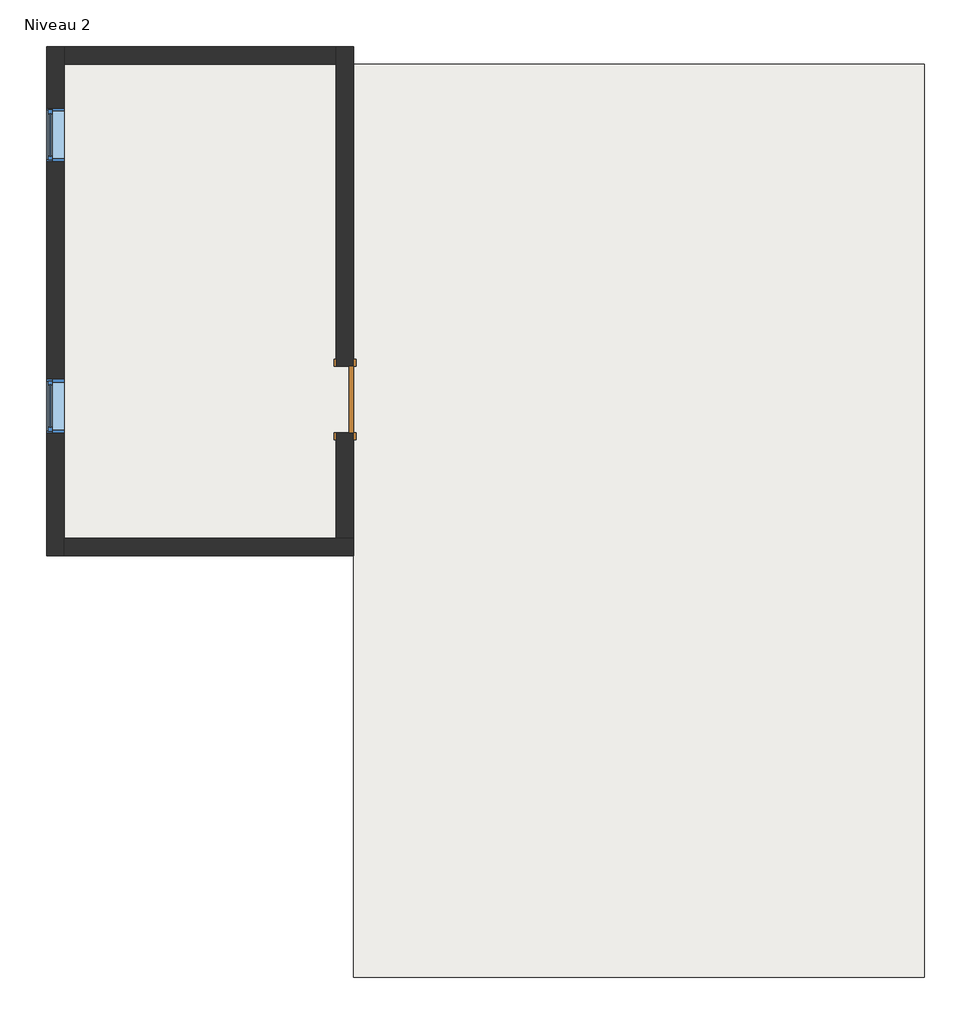
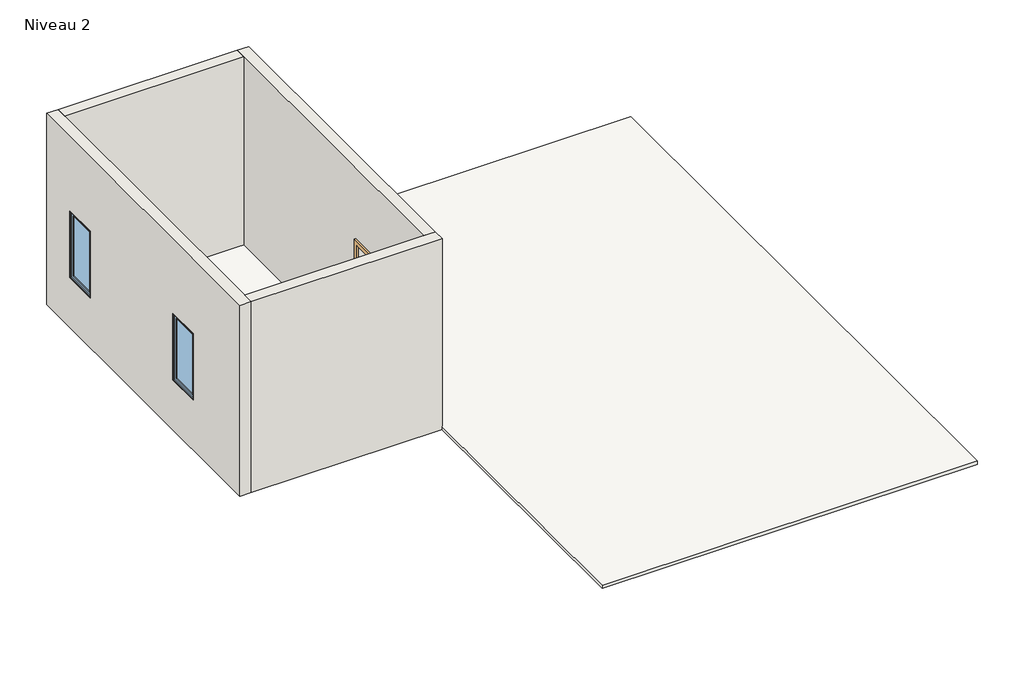
# One storey: 4 walls, 2 windows, 1 covering, 1 door.
"""IFC4 building model written with IfcOpenShell, lengths in millimetres."""

import ifcopenshell
import ifcopenshell.guid

model = None  # the IFC model being written
_history = None  # IfcOwnerHistory: only IFC2X3 demands one
_inside = {}  # id of a spatial element -> (the spatial element, [elements in it])
_under = {}  # id of a project, library or spatial element -> (it, [spatial elements below it])
_declared = {}  # id of a project -> (the project, [libraries it declares])
_typed = {}  # id of a type object -> (the type object, [elements of that type])
_made_of = {}  # id of a material, layer set ... -> (it, [elements and type objects made of it])


def new_model(schema):
    """Start an empty IFC model of exactly this schema.

    Asked for "IFC4X3", IfcOpenShell would pick the latest addendum, in which some entities
    have other attributes; the version numbers below select the first issue.
    IFC2X3 requires an IfcOwnerHistory on every rooted entity: one is made here for all.
    """
    global model, _history
    if schema == "IFC4X3":
        model = ifcopenshell.file(schema_version=(4, 3, 0, 0))
    else:
        model = ifcopenshell.file(schema=schema)
    _inside.clear()
    _under.clear()
    _declared.clear()
    _typed.clear()
    _made_of.clear()
    _history = None
    if model.schema == "IFC2X3":
        org = make("IfcOrganization", Name="unknown")
        user = make(
            "IfcPersonAndOrganization",
            ThePerson=make("IfcPerson", FamilyName="unknown"),
            TheOrganization=org,
        )
        app = make(
            "IfcApplication",
            ApplicationDeveloper=org,
            Version="unknown",
            ApplicationFullName="unknown",
            ApplicationIdentifier="unknown",
        )
        _history = make(
            "IfcOwnerHistory",
            OwningUser=user,
            OwningApplication=app,
            ChangeAction="ADDED",
            CreationDate=0,
        )
    return model


def make(cls, **values):
    """One entity of the class cls with the attributes given. An attribute that is None is left unset."""
    return model.create_entity(
        cls, **{name: value for name, value in values.items() if value is not None}
    )


def rooted(cls, **values):
    """An entity with a GlobalId (a new one), such as an element, a storey or a relation."""
    return make(cls, GlobalId=ifcopenshell.guid.new(), OwnerHistory=_history, **values)


def si_unit(unit_type, name, prefix=None):
    """IfcSIUnit, for example si_unit("LENGTHUNIT", "METRE", prefix="MILLI")."""
    return make("IfcSIUnit", UnitType=unit_type, Prefix=prefix, Name=name)


def assignment(units):
    """IfcUnitAssignment: the units of a project."""
    return None if units is None else make("IfcUnitAssignment", Units=units)


def point(xyz):
    """IfcCartesianPoint."""
    return None if xyz is None else make("IfcCartesianPoint", Coordinates=xyz)


def direction(xyz):
    """IfcDirection."""
    return None if xyz is None else make("IfcDirection", DirectionRatios=xyz)


def frame(location, z_axis=None, x_axis=None):
    """IfcAxis2Placement3D, a coordinate frame: its origin and axes. An axis left out is left unset."""
    return make(
        "IfcAxis2Placement3D",
        Location=point(location),
        Axis=direction(z_axis),
        RefDirection=direction(x_axis),
    )


def origin():
    """The frame at (0, 0, 0) with its axes left unset."""
    return frame((0.0, 0.0, 0.0))


def origin_with_axes():
    """The frame at (0, 0, 0) with the z axis (0, 0, 1) and the x axis (1, 0, 0) written out."""
    return frame((0.0, 0.0, 0.0), z_axis=(0.0, 0.0, 1.0), x_axis=(1.0, 0.0, 0.0))


def place(relative_to, where):
    """IfcLocalPlacement: puts the frame where relative to a parent placement (None: the world)."""
    return make(
        "IfcLocalPlacement", PlacementRelTo=relative_to, RelativePlacement=where
    )


def context(
    kind, dimensions, precision=None, world=None, true_north=None, identifier=None
):
    """IfcGeometricRepresentationContext, for example the 3D "Model" context."""
    return make(
        "IfcGeometricRepresentationContext",
        ContextIdentifier=identifier,
        ContextType=kind,
        CoordinateSpaceDimension=dimensions,
        Precision=precision,
        WorldCoordinateSystem=world,
        TrueNorth=true_north,
    )


def project(units=None, contexts=None):
    """IfcProject with its units and contexts."""
    return rooted(
        "IfcProject",
        Name="project",
        RepresentationContexts=contexts,
        UnitsInContext=assignment(units),
    )


def spatial(cls, under=None, at=None, **own):
    """A site, building, storey or space (cls), placed at a placement, below another one or the project."""
    s = rooted(cls, ObjectPlacement=at, **own)
    if under is not None:
        _under.setdefault(under.id(), (under, []))[1].append(s)
    return s


def polyline(points):
    """IfcPolyline through the points."""
    return make("IfcPolyline", Points=[point(p) for p in points])


def outline(outer, holes=None, kind="AREA"):
    """IfcArbitraryClosedProfileDef: a profile drawn as a closed curve; with holes, ...WithVoids."""
    if holes is None:
        return make("IfcArbitraryClosedProfileDef", ProfileType=kind, OuterCurve=outer)
    return make(
        "IfcArbitraryProfileDefWithVoids",
        ProfileType=kind,
        OuterCurve=outer,
        InnerCurves=holes,
    )


def extrude(swept, where, along, depth):
    """IfcExtrudedAreaSolid: the profile swept, set in the frame where, extruded along a direction by depth."""
    return make(
        "IfcExtrudedAreaSolid",
        SweptArea=swept,
        Position=where,
        ExtrudedDirection=direction(along),
        Depth=depth,
    )


def faces_of(points, faces, orient=None, outer=None):
    """IfcFace entities. A face is a list of loops; a loop is a list of indices into points, from 0.

    orient and outer hold one flag for each loop. By default every Orientation is true, the
    first loop of a face is its IfcFaceOuterBound and the others are IfcFaceBound.
    """
    made = []
    for i, loops in enumerate(faces):
        bounds = []
        for j, loop in enumerate(loops):
            is_outer = j == 0 if outer is None else outer[i][j]
            bounds.append(
                make(
                    "IfcFaceOuterBound" if is_outer else "IfcFaceBound",
                    Bound=make("IfcPolyLoop", Polygon=[points[k] for k in loop]),
                    Orientation=True if orient is None else orient[i][j],
                )
            )
        made.append(make("IfcFace", Bounds=bounds))
    return made


def faceted_brep(points, faces, orient=None, outer=None, voids=None):
    """IfcFacetedBrep: a solid bounded by flat faces; with voids (closed shells), ...WithVoids."""
    shared = [point(p) for p in points]
    hull = make("IfcClosedShell", CfsFaces=faces_of(shared, faces, orient, outer))
    if voids is None:
        return make("IfcFacetedBrep", Outer=hull)
    return make(
        "IfcFacetedBrepWithVoids",
        Outer=hull,
        Voids=[
            make(cls, CfsFaces=faces_of(shared, fs, o, b)) for cls, fs, o, b in voids
        ],
    )


def shape(context_of_items, identifier, shape_type, items):
    """IfcShapeRepresentation: the items that make up one representation, for example the "Body"."""
    return make(
        "IfcShapeRepresentation",
        ContextOfItems=context_of_items,
        RepresentationIdentifier=identifier,
        RepresentationType=shape_type,
        Items=items,
    )


def source(mapping_origin, context_of_items, identifier, shape_type, items):
    """IfcRepresentationMap: a shape defined once, which mapped items show again and again."""
    return make(
        "IfcRepresentationMap",
        MappingOrigin=mapping_origin,
        MappedRepresentation=shape(context_of_items, identifier, shape_type, items),
    )


def transform(
    local_origin,
    x_axis=None,
    y_axis=None,
    z_axis=None,
    scale=None,
    scale2=None,
    scale3=None,
    uniform=True,
):
    """IfcCartesianTransformationOperator3D, or its non-uniform kind. x_axis, y_axis, z_axis: its Axis1, 2, 3."""
    if uniform:
        return make(
            "IfcCartesianTransformationOperator3D",
            Axis1=direction(x_axis),
            Axis2=direction(y_axis),
            LocalOrigin=point(local_origin),
            Scale=scale,
            Axis3=direction(z_axis),
        )
    return make(
        "IfcCartesianTransformationOperator3DnonUniform",
        Axis1=direction(x_axis),
        Axis2=direction(y_axis),
        LocalOrigin=point(local_origin),
        Scale=scale,
        Axis3=direction(z_axis),
        Scale2=scale2,
        Scale3=scale3,
    )


def mapped(mapping_source, mapping_target):
    """IfcMappedItem: shows the shape of a source again, moved by a transform."""
    return make(
        "IfcMappedItem", MappingSource=mapping_source, MappingTarget=mapping_target
    )


def made_of(thing, what):
    """Note that an element or type object is made of a material, layer set ...; save() writes the relation."""
    if what is not None:
        _made_of.setdefault(what.id(), (what, []))[1].append(thing)
    return thing


def element(
    cls,
    number,
    at=None,
    inside=None,
    cuts=None,
    type_object=None,
    material=None,
    context=None,
    identifier="Body",
    shape_type=None,
    held_by="IfcProductDefinitionShape",
    body=None,
    shapes=None,
    **own,
):
    """One element of the class cls, such as IfcWall. Its Tag is "e" and its number.

    at: its placement. inside: the storey or other place that contains it. cuts: it is an
    opening in that element (IfcRelVoidsElement). A single representation is given by context,
    identifier, shape_type and body (its items); several are given by shapes. held_by: the class
    of the entity that holds the representations. save() writes the other relations.
    """
    e = rooted(cls, Tag="e%d" % number, ObjectPlacement=at, **own)
    if body is not None:
        shapes = [shape(context, identifier, shape_type, body)]
    if shapes is not None:
        e.Representation = make(held_by, Representations=shapes)
    if inside is not None:
        _inside.setdefault(inside.id(), (inside, []))[1].append(e)
    if cuts is not None:
        rooted(
            "IfcRelVoidsElement", RelatingBuildingElement=cuts, RelatedOpeningElement=e
        )
    if type_object is not None:
        _typed.setdefault(type_object.id(), (type_object, []))[1].append(e)
    return made_of(e, material)


def aggregate(whole, parts):
    """IfcRelAggregates: a whole, such as a stair, and the parts it consists of."""
    return rooted("IfcRelAggregates", RelatingObject=whole, RelatedObjects=parts)


def save(model, path):
    """Write the relations noted so far, then the file.

    IfcRelAggregates (storeys below a building ...), IfcRelContainedInSpatialStructure (elements
    in a storey), IfcRelDefinesByType, IfcRelAssociatesMaterial and IfcRelDeclares: one each for
    every whole, place, type object, material and project.
    """
    for whole, parts in _under.values():
        aggregate(whole, parts)
    for where, things in _inside.values():
        rooted(
            "IfcRelContainedInSpatialStructure",
            RelatedElements=things,
            RelatingStructure=where,
        )
    for kind, things in _typed.values():
        rooted("IfcRelDefinesByType", RelatedObjects=things, RelatingType=kind)
    for what, things in _made_of.values():
        rooted("IfcRelAssociatesMaterial", RelatedObjects=things, RelatingMaterial=what)
    for by, libraries in _declared.values():
        rooted("IfcRelDeclares", RelatingContext=by, RelatedDefinitions=libraries)
    model.write(path)


def simple_avec_alignement_0762_x_2134mm_85379237(model_context):
    return source(origin(), model_context, "Body", "SweptSolid", [
        extrude(outline(polyline([(2210.0, -457.0), (0.0, -457.0), (0.0, -381.0), (2134.0, -381.0), (2134.0, 381.0), (0.0, 381.0), (0.0, 457.0), (2210.0, 457.0), (2210.0, -457.0)])), frame((0.0, 100.0, 0.0), z_axis=(0.0, 1.0, 0.0), x_axis=(0.0, 0.0, 1.0)), (0.0, 0.0, 1.0), 25.0),
        extrude(outline(polyline([(2210.0, 457.0), (2210.0, -457.0), (0.0, -457.0), (0.0, -381.0), (2134.0, -381.0), (2134.0, 381.0), (0.0, 381.0), (0.0, 457.0), (2210.0, 457.0)])), frame((0.0, -125.0, 0.0), z_axis=(0.0, 1.0, 0.0), x_axis=(0.0, 0.0, 1.0)), (0.0, 0.0, 1.0), 25.0),
        extrude(outline(polyline([(381.0, 49.0), (-381.0, 49.0), (-381.0, 100.0), (381.0, 100.0), (381.0, 49.0)])), origin_with_axes(), (0.0, 0.0, 1.0), 2134.0),
    ])


def fixe_0610_x_1220mm_4e981104(model_context):
    return source(origin(), model_context, "Body", "SweptSolid", [
        extrude(outline(polyline([(-242.0, 78.0), (242.0, 78.0), (242.0, 66.0), (-242.0, 66.0), (-242.0, 78.0)])), frame((0.0, 0.0, 978.0), z_axis=(0.0, 0.0, 1.0), x_axis=(1.0, 0.0, 0.0)), (0.0, 0.0, 1.0), 1094.0),
        extrude(outline(polyline([(2116.0, -286.0), (934.0, -286.0), (934.0, 286.0), (2116.0, 286.0), (2116.0, -286.0)]), holes=[polyline([(2072.0, -242.0), (2072.0, 242.0), (978.0, 242.0), (978.0, -242.0), (2072.0, -242.0)])]), frame((0.0, 50.0, 0.0), z_axis=(0.0, 1.0, 0.0), x_axis=(0.0, 0.0, 1.0)), (0.0, 0.0, 1.0), 44.0),
        extrude(outline(polyline([(2135.0, -305.0), (915.0, -305.0), (915.0, 305.0), (2135.0, 305.0), (2135.0, -305.0)]), holes=[polyline([(2116.0, -286.0), (2116.0, 286.0), (934.0, 286.0), (934.0, -286.0), (2116.0, -286.0)])]), frame((0.0, 50.0, 0.0), z_axis=(0.0, 1.0, 0.0), x_axis=(0.0, 0.0, 1.0)), (0.0, 0.0, 1.0), 63.0),
        extrude(outline(polyline([(2135.0, -305.0), (915.0, -305.0), (915.0, 305.0), (2135.0, 305.0), (2135.0, -305.0)]), holes=[polyline([(2103.0, -273.0), (2103.0, 273.0), (947.0, 273.0), (947.0, -273.0), (2103.0, -273.0)])]), frame((0.0, -87.0, 0.0), z_axis=(0.0, 1.0, 0.0), x_axis=(0.0, 0.0, 1.0)), (0.0, 0.0, 1.0), 137.0),
    ])


model = new_model("IFC4")

# Units and contexts
model_context = context("Model", 3, world=origin())
ifc_project = project(units=[si_unit("LENGTHUNIT", "METRE", prefix="MILLI")], contexts=[model_context])

# Site, building, storey
site = spatial("IfcSite", under=ifc_project)
building = spatial("IfcBuilding", under=site)
storey = spatial("IfcBuildingStorey", under=building, Name="Niveau 2", Elevation=4000.0)

# Covering
placement = place(None, origin())
element("IfcCovering", 1, ObjectType="Normal", at=placement, inside=storey, context=model_context, shape_type="SweptSolid", body=[
    extrude(outline(polyline([(-4921.6723283, -1160.6445533), (-4921.6723283, 4239.3554467), (4878.3276717, 4239.3554467), (4878.3276717, -6160.6445533), (-1621.6723283, -6160.6445533), (-1621.6723283, -1160.6445533), (-4921.6723283, -1160.6445533)])), frame((0.0, 0.0, 4000.0), z_axis=(0.0, 0.0, 1.0), x_axis=(1.0, 0.0, 0.0)), (0.0, 0.0, 1.0), 57.0),
])

# Door
simple_avec_alignement_0762_x_2134mm_shape = simple_avec_alignement_0762_x_2134mm_85379237(model_context)
element("IfcDoor", 2, ObjectType="Simple avec alignement : 0762 x 2134mm", at=placement, inside=storey, context=model_context, shape_type="MappedRepresentation", body=[
    mapped(simple_avec_alignement_0762_x_2134mm_shape, transform((-1721.6723283, 420.3554467, 4000.0), x_axis=(0.0, -1.0, 0.0), y_axis=(1.0, 0.0, 0.0), z_axis=(0.0, 0.0, 1.0))),
])

# Walls
element("IfcWall", 3, ObjectType="Générique - 200 mm", at=placement, inside=storey, context=model_context, shape_type="Brep", body=[
    faceted_brep([(-5121.6723283, 4439.3554467, 4000.0), (-5121.6723283, -1360.6445533, 4000.0), (-5121.6723283, -1360.6445533, 7500.0), (-5121.6723283, 4439.3554467, 7500.0), (-5121.6723283, 3129.3554467, 4915.0), (-5121.6723283, 3739.3554467, 4915.0), (-5121.6723283, 3739.3554467, 6135.0), (-5121.6723283, 3129.3554467, 6135.0), (-5121.6723283, 39.3554467, 4915.0), (-5121.6723283, 649.3554467, 4915.0), (-5121.6723283, 649.3554467, 6135.0), (-5121.6723283, 39.3554467, 6135.0), (-4921.6723283, 4439.3554467, 4000.0), (-4921.6723283, 4439.3554467, 7500.0), (-4921.6723283, 4239.3554467, 7500.0), (-4921.6723283, -1160.6445533, 7500.0), (-4921.6723283, -1360.6445533, 7500.0), (-4921.6723283, -1360.6445533, 4000.0), (-4921.6723283, -1160.6445533, 4000.0), (-4921.6723283, 4239.3554467, 4000.0), (-4921.6723283, 3129.3554467, 4915.0), (-4921.6723283, 3129.3554467, 6135.0), (-4921.6723283, 3739.3554467, 6135.0), (-4921.6723283, 3739.3554467, 4915.0), (-4921.6723283, 39.3554467, 4915.0), (-4921.6723283, 39.3554467, 6135.0), (-4921.6723283, 649.3554467, 6135.0), (-4921.6723283, 649.3554467, 4915.0)], [[[0, 1, 2, 3], [4, 5, 6, 7], [8, 9, 10, 11]], [[12, 13, 14, 15, 16, 17, 18, 19], [20, 21, 22, 23], [24, 25, 26, 27]], [[1, 0, 12, 19, 18, 17]], [[3, 2, 16, 15, 14, 13]], [[2, 1, 17, 16]], [[0, 3, 13, 12]], [[21, 20, 4, 7]], [[22, 21, 7, 6]], [[23, 22, 6, 5]], [[20, 23, 5, 4]], [[25, 24, 8, 11]], [[26, 25, 11, 10]], [[27, 26, 10, 9]], [[24, 27, 9, 8]]]),
])
element("IfcWall", 4, ObjectType="Générique - 200 mm", at=placement, inside=storey, context=model_context, shape_type="Brep", body=[
    faceted_brep([(-4921.6723283, -1360.6445533, 4000.0), (-1621.6723283, -1360.6445533, 4000.0), (-1621.6723283, -1360.6445533, 7500.0), (-4921.6723283, -1360.6445533, 7500.0), (-4921.6723283, -1160.6445533, 4000.0), (-4921.6723283, -1160.6445533, 7500.0), (-1821.6723283, -1160.6445533, 7500.0), (-1621.6723283, -1160.6445533, 7500.0), (-1621.6723283, -1160.6445533, 4000.0), (-1821.6723283, -1160.6445533, 4000.0)], [[[0, 1, 2, 3]], [[4, 5, 6, 7, 8, 9]], [[1, 0, 4, 9, 8]], [[3, 2, 7, 6, 5]], [[0, 3, 5, 4]], [[2, 1, 8, 7]]]),
])
element("IfcWall", 5, ObjectType="Générique - 200 mm", at=placement, inside=storey, context=model_context, shape_type="Brep", body=[
    faceted_brep([(-1621.6723283, -1160.6445533, 4000.0), (-1621.6723283, 39.3554467, 4000.0), (-1621.6723283, 39.3554467, 6134.0), (-1621.6723283, 801.3554467, 6134.0), (-1621.6723283, 801.3554467, 4000.0), (-1621.6723283, 4439.3554467, 4000.0), (-1621.6723283, 4439.3554467, 7500.0), (-1621.6723283, -1160.6445533, 7500.0), (-1821.6723283, 39.3554467, 6134.0), (-1821.6723283, 39.3554467, 4000.0), (-1821.6723283, -1160.6445533, 4000.0), (-1821.6723283, -1160.6445533, 7500.0), (-1821.6723283, 4239.3554467, 7500.0), (-1821.6723283, 4439.3554467, 7500.0), (-1821.6723283, 4439.3554467, 4000.0), (-1821.6723283, 4239.3554467, 4000.0), (-1821.6723283, 801.3554467, 4000.0), (-1821.6723283, 801.3554467, 6134.0)], [[[0, 1, 2, 3, 4, 5, 6, 7]], [[8, 9, 10, 11, 12, 13, 14, 15, 16, 17]], [[10, 9, 1, 0]], [[16, 15, 14, 5, 4]], [[7, 6, 13, 12, 11]], [[0, 7, 11, 10]], [[6, 5, 14, 13]], [[2, 1, 9, 8]], [[3, 2, 8, 17]], [[4, 3, 17, 16]]]),
])
element("IfcWall", 6, ObjectType="Générique - 200 mm", at=placement, inside=storey, context=model_context, shape_type="SweptSolid", body=[
    extrude(outline(polyline([(-4921.6723283, 4439.3554467), (-1821.6723283, 4439.3554467), (-1821.6723283, 4239.3554467), (-4921.6723283, 4239.3554467), (-4921.6723283, 4439.3554467)])), frame((0.0, 0.0, 4000.0), z_axis=(0.0, 0.0, 1.0), x_axis=(1.0, 0.0, 0.0)), (0.0, 0.0, 1.0), 3500.0),
])

# Windows
fixe_0610_x_1220mm_shape = fixe_0610_x_1220mm_4e981104(model_context)
element("IfcWindow", 7, ObjectType="Fixe : 0610 x 1220mm", at=placement, inside=storey, context=model_context, shape_type="MappedRepresentation", body=[
    mapped(fixe_0610_x_1220mm_shape, transform((-5008.6723283, 3434.3554467, 4000.0), x_axis=(0.0, 1.0, 0.0), y_axis=(-1.0, 0.0, 0.0), z_axis=(0.0, 0.0, 1.0))),
])
element("IfcWindow", 8, ObjectType="Fixe : 0610 x 1220mm", at=placement, inside=storey, context=model_context, shape_type="MappedRepresentation", body=[
    mapped(fixe_0610_x_1220mm_shape, transform((-5008.6723283, 344.3554467, 4000.0), x_axis=(0.0, 1.0, 0.0), y_axis=(-1.0, 0.0, 0.0), z_axis=(0.0, 0.0, 1.0))),
])

save(model, "model.ifc")

# Revit data of these elements
# Type "Normal"
#   built-in parameter 1002203 = 1 (stored number, unit not read)
#   built-in parameter 1002202 = 1 (stored number, unit not read)
#   Layers, outside or top first: 0.045 m "Montant métallique" (function 1); 0.012 m "Plaque de mur de gypse" (function 5)
# Type "Simple avec alignement : 0762 x 2134mm"
#   Type Mark = "16"
#   Construction Type Id = "MDOOR"
#   Analytic Construction = "Métal"
#   Thickness = 0.051 m
#   Heat Transfer Coefficient (U) = 3.7021 W/(m²·K)
#   Height = 2.134 m
#   Ajuster la projection Ext = 0.025 m
#   Ajuster la projection Int = 0.025 m
#   Ajuster la largeur = 0.076 m
#   Width = 0.762 m
#   Function = 0
#   Define Thermal Properties by = 1
#   Matériau de porte = Porte - Panneau
#   Matériau des huisseries = Porte - Cadre
#   Visual Light Transmittance = 0
#   Solar Heat Gain Coefficient = 0
#   Function = (empty or 0)
#   Wall Closure = (empty or 0)
# Type "Générique - 200 mm"
#   Layers, outside or top first: 0.20 m no material (function 1)
# Type "Fixe : 0610 x 1220mm"
#   Type Mark = "13"
#   Construction Type Id = "GSP4R"
#   Analytic Construction = "Simple vitrage Pilkington 1/8 po."
#   Visual Light Transmittance = 0.9
#   Solar Heat Gain Coefficient = 0.78
#   Heat Transfer Coefficient (U) = 3.6886 W/(m²·K)
#   Height = 1.22 m
#   Hauteur de l'appui par défaut = 0.915 m
#   Width = 0.61 m
#   Encastrement de fenêtre = 0.019 m
#   Define Thermal Properties by = 1
#   Matériau de cadre extérieur = Châssis
#   Matériau du cadre intérieur = Châssis
#   Matériau du panneau de verre = Verre
#   Châssis = Châssis
#   Wall Closure = (empty or 0)
# Element 1 (IfcCovering, "Normal")
#   Height Offset From Level = 0.00 m
#   Cout total = 546445
#   Cout unitaire = 10
#   Phase Created = Phase 1
#   Materials on its faces: "Plaque de mur de gypse", "Montant métallique"
# Element 2 (IfcDoor, "Simple avec alignement : 0762 x 2134mm")
#   Phase Created = Phase 1
#   Materials on its faces: "Porte - Cadre", "Porte - Panneau"
# Elements 3, 4, 5, 6 (IfcWall, "Générique - 200 mm")
#   Top Offset = 0.00 m
#   Base Offset = 0.00 m
#   wall height = 3.50 m
#   Phase Created = Phase 1
#   Base Constraint = Niveau 2
#   Top Constraint = Niveau 3
#   Materials on its faces: "Mur par défaut"
# Element 7 (IfcWindow, "Fixe : 0610 x 1220mm")
#   Mark = "6"
#   Phase Created = Phase 1
#   Materials on its faces: "Châssis", "Verre"
# Element 8 (IfcWindow, "Fixe : 0610 x 1220mm")
#   Mark = "7"
#   Phase Created = Phase 1
#   Materials on its faces: "Châssis", "Verre"
# Materials
#   "Montant métallique": class "Métal", colour RGB 127 127 127, transparency 0, Description = "Poutre en acier léger, couche isolante/lame d'air", Cost = 0
#   "Plaque de mur de gypse": class "Générique", colour RGB 249 249 249, transparency 0, Description = "Plaque de mur de gypse", Cost = 0
#   "Porte - Panneau": class "Bois", colour RGB 210 159 95, transparency 0, Cost = 0
#   "Porte - Cadre": class "Peinture", colour RGB 118 70 51, transparency 0, Cost = 0
#   "Châssis": class "Bois", colour RGB 224 178 126, transparency 0, Cost = 0
#   "Verre": class "Verre", colour RGB 0 128 192, transparency 0.9, Description = "Verre sodocalcique", Cost = 0
#   "Mur par défaut": class "Divers", colour RGB 128 128 128, transparency 0, Cost = 0
